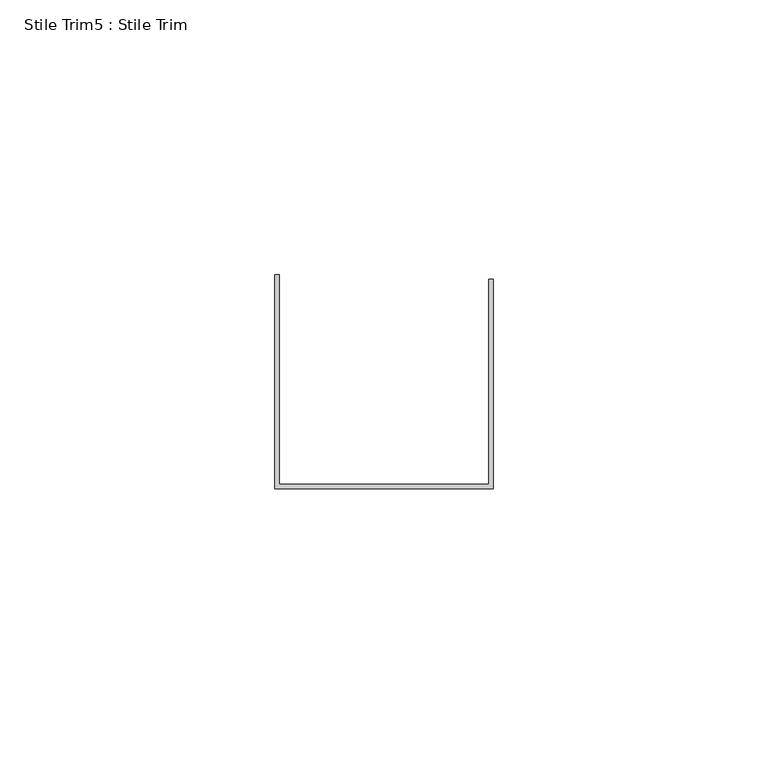
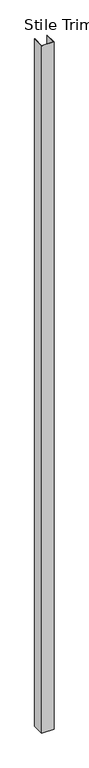
"""IFC4 building model written with IfcOpenShell, lengths in millimetres: proxy geometry, Stile Trim5 : Stile Trim."""

from ifc_helpers import new_model, si_unit, frame, origin, place, context, project, spatial, polyline, outline, extrude, source, transform, mapped, element, save


def stile_trim5_stile_trim_35358b3a(model_context):
    return source(origin(), model_context, "Body", "SweptSolid", [
        extrude(outline(polyline([(587327.0060739, -532878.2537841), (587327.0060739, -532839.3663841), (587327.7934739, -532839.3663841), (587327.7934739, -532877.4663841), (587365.8934739, -532877.4663841), (587365.8934739, -532840.1537841), (587366.6808739, -532840.1537841), (587366.6808739, -532878.2537841), (587327.0060739, -532878.2537841)])), frame((0.0, 0.0, 50.8), z_axis=(0.0, 0.0, 1.0), x_axis=(1.0, 0.0, 0.0)), (0.0, 0.0, 1.0), 2350.3929688),
    ])


if __name__ == "__main__":
    model = new_model("IFC4")
    model_context = context("Model", 3, world=origin())
    ifc_project = project(units=[si_unit("LENGTHUNIT", "METRE", prefix="MILLI")], contexts=[model_context])
    site = spatial("IfcSite", under=ifc_project)
    building = spatial("IfcBuilding", under=site)
    placement = place(None, origin())
    stile_trim5_stile_trim_shape = stile_trim5_stile_trim_35358b3a(model_context)
    element("IfcBuildingElementProxy", 1, Name="Stile Trim5 : Stile Trim", ObjectType="Stile Trim5 : Stile Trim", at=placement, inside=building, context=model_context, shape_type="MappedRepresentation", body=[
        mapped(stile_trim5_stile_trim_shape, transform((0.0, 0.0, 0.0), x_axis=(1.0, 0.0, 0.0), y_axis=(0.0, 1.0, 0.0), z_axis=(0.0, 0.0, 1.0))),
    ])
    save(model, "model.ifc")

# Revit data of these elements
# Element 1 (IfcBuildingElementProxy, "Stile Trim5 : Stile Trim")
#   Materials on its faces: "EDGE TRIM BY MTL PANEL MFR."
# Materials
#   "EDGE TRIM BY MTL PANEL MFR.": class "Generic", colour RGB 239 242 240, transparency 0, Cost = 0
